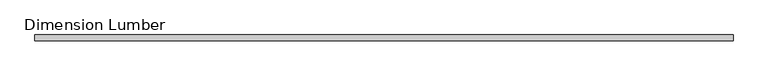
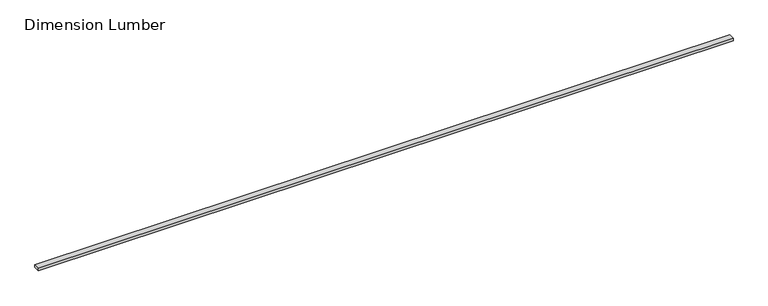
"""IFC4 building model written with IfcOpenShell, lengths in millimetres: beam geometry, Dimension Lumber : Top Supporting Lumbers."""

from ifc_helpers import new_model, si_unit, frame, origin, place, context, project, spatial, polyline, outline, extrude, source, transform, mapped, element, save


def dimension_lumber_c8f8d63a(model_context):
    return source(origin(), model_context, "Body", "SweptSolid", [
        extrude(outline(polyline([(5118.89375, 44.45), (5118.89375, -44.45), (-5118.89375, -44.45), (-5118.89375, 44.45), (5118.89375, 44.45)])), frame((0.0, 0.0, -19.05), z_axis=(0.0, 0.0, 1.0), x_axis=(1.0, 0.0, 0.0)), (0.0, 0.0, 1.0), 38.1),
    ])


if __name__ == "__main__":
    model = new_model("IFC4")
    model_context = context("Model", 3, world=origin())
    ifc_project = project(units=[si_unit("LENGTHUNIT", "METRE", prefix="MILLI")], contexts=[model_context])
    site = spatial("IfcSite", under=ifc_project)
    building = spatial("IfcBuilding", under=site)
    placement = place(None, origin())
    dimension_lumber_shape = dimension_lumber_c8f8d63a(model_context)
    element("IfcBeam", 1, ObjectType="Dimension Lumber : Top Supporting Lumbers", at=placement, inside=building, context=model_context, shape_type="MappedRepresentation", body=[
        mapped(dimension_lumber_shape, transform((0.0, 0.0, 0.0), x_axis=(1.0, 0.0, 0.0), y_axis=(0.0, 1.0, 0.0), z_axis=(0.0, 0.0, 1.0))),
    ])
    save(model, "model.ifc")

# Revit data of these elements
# Type "Dimension Lumber : Top Supporting Lumbers"
#   Assembly Code = "B10"
#   A = 0.0364583 SF
#   Length [instance default] = 5' - 0"
#   b = 0' - 3 1/2"
#   d = 0' - 1 1/2"
#   Structural Material [instance default] = Softwood, Lumber
# Element 1 (IfcBeam, "Dimension Lumber : Top Supporting Lumbers")
#   Structural Material = Douglas Fir #2
#   Materials on its faces: "Douglas Fir #2"
# Materials
#   "Softwood, Lumber": class "Wood", colour RGB 223 192 134, transparency 0, Description = "Pinus Echinata", Cost = 0
#   "Douglas Fir #2": class "Wood", colour RGB 223 192 134, transparency 0, Description = "Pinus Echinata", Cost = 0
